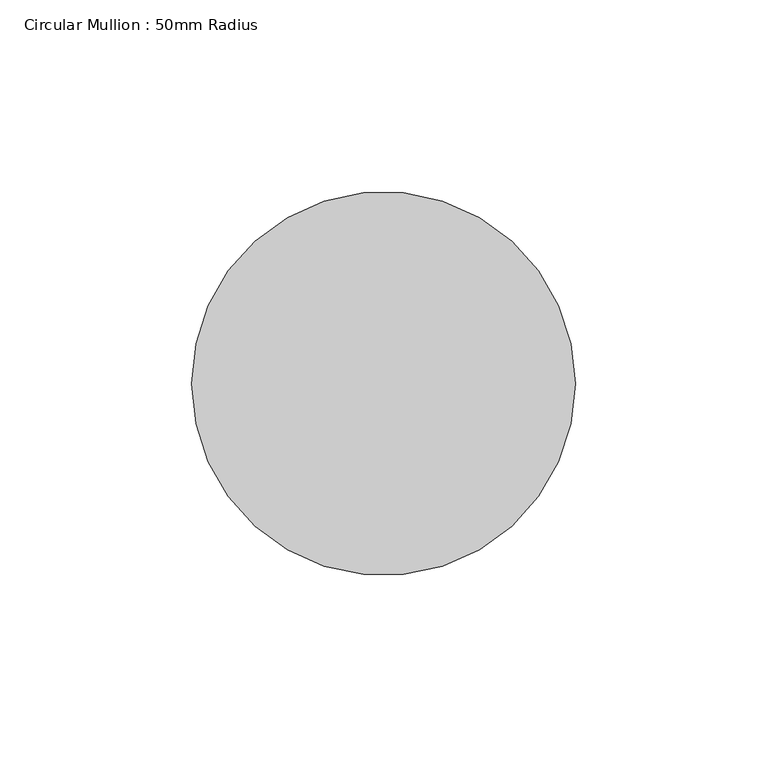
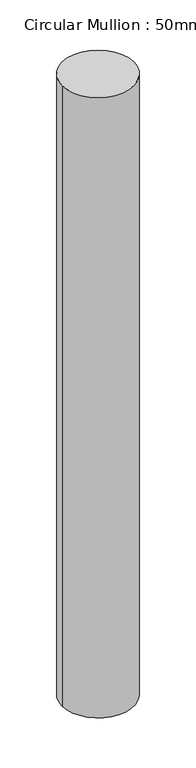
"""IFC4 building model written with IfcOpenShell, lengths in millimetres: member geometry, Circular Mullion : 50mm Radius."""

import ifcopenshell
import ifcopenshell.guid

model = None  # the IFC model being written
_history = None  # IfcOwnerHistory: only IFC2X3 demands one
_inside = {}  # id of a spatial element -> (the spatial element, [elements in it])
_under = {}  # id of a project, library or spatial element -> (it, [spatial elements below it])
_declared = {}  # id of a project -> (the project, [libraries it declares])
_typed = {}  # id of a type object -> (the type object, [elements of that type])
_made_of = {}  # id of a material, layer set ... -> (it, [elements and type objects made of it])


def new_model(schema):
    """Start an empty IFC model of exactly this schema.

    Asked for "IFC4X3", IfcOpenShell would pick the latest addendum, in which some entities
    have other attributes; the version numbers below select the first issue.
    IFC2X3 requires an IfcOwnerHistory on every rooted entity: one is made here for all.
    """
    global model, _history
    if schema == "IFC4X3":
        model = ifcopenshell.file(schema_version=(4, 3, 0, 0))
    else:
        model = ifcopenshell.file(schema=schema)
    _inside.clear()
    _under.clear()
    _declared.clear()
    _typed.clear()
    _made_of.clear()
    _history = None
    if model.schema == "IFC2X3":
        org = make("IfcOrganization", Name="unknown")
        user = make(
            "IfcPersonAndOrganization",
            ThePerson=make("IfcPerson", FamilyName="unknown"),
            TheOrganization=org,
        )
        app = make(
            "IfcApplication",
            ApplicationDeveloper=org,
            Version="unknown",
            ApplicationFullName="unknown",
            ApplicationIdentifier="unknown",
        )
        _history = make(
            "IfcOwnerHistory",
            OwningUser=user,
            OwningApplication=app,
            ChangeAction="ADDED",
            CreationDate=0,
        )
    return model


def make(cls, **values):
    """One entity of the class cls with the attributes given. An attribute that is None is left unset."""
    return model.create_entity(
        cls, **{name: value for name, value in values.items() if value is not None}
    )


def rooted(cls, **values):
    """An entity with a GlobalId (a new one), such as an element, a storey or a relation."""
    return make(cls, GlobalId=ifcopenshell.guid.new(), OwnerHistory=_history, **values)


def si_unit(unit_type, name, prefix=None):
    """IfcSIUnit, for example si_unit("LENGTHUNIT", "METRE", prefix="MILLI")."""
    return make("IfcSIUnit", UnitType=unit_type, Prefix=prefix, Name=name)


def assignment(units):
    """IfcUnitAssignment: the units of a project."""
    return None if units is None else make("IfcUnitAssignment", Units=units)


def point(xyz):
    """IfcCartesianPoint."""
    return None if xyz is None else make("IfcCartesianPoint", Coordinates=xyz)


def direction(xyz):
    """IfcDirection."""
    return None if xyz is None else make("IfcDirection", DirectionRatios=xyz)


def frame(location, z_axis=None, x_axis=None):
    """IfcAxis2Placement3D, a coordinate frame: its origin and axes. An axis left out is left unset."""
    return make(
        "IfcAxis2Placement3D",
        Location=point(location),
        Axis=direction(z_axis),
        RefDirection=direction(x_axis),
    )


def frame_2d(location, x_axis=None):
    """IfcAxis2Placement2D, a coordinate frame in the plane: its origin and x axis."""
    return make(
        "IfcAxis2Placement2D", Location=point(location), RefDirection=direction(x_axis)
    )


def origin():
    """The frame at (0, 0, 0) with its axes left unset."""
    return frame((0.0, 0.0, 0.0))


def origin_2d():
    """The frame at (0, 0) in the plane with its x axis left unset."""
    return frame_2d((0.0, 0.0))


def place(relative_to, where):
    """IfcLocalPlacement: puts the frame where relative to a parent placement (None: the world)."""
    return make(
        "IfcLocalPlacement", PlacementRelTo=relative_to, RelativePlacement=where
    )


def context(
    kind, dimensions, precision=None, world=None, true_north=None, identifier=None
):
    """IfcGeometricRepresentationContext, for example the 3D "Model" context."""
    return make(
        "IfcGeometricRepresentationContext",
        ContextIdentifier=identifier,
        ContextType=kind,
        CoordinateSpaceDimension=dimensions,
        Precision=precision,
        WorldCoordinateSystem=world,
        TrueNorth=true_north,
    )


def project(units=None, contexts=None):
    """IfcProject with its units and contexts."""
    return rooted(
        "IfcProject",
        Name="project",
        RepresentationContexts=contexts,
        UnitsInContext=assignment(units),
    )


def spatial(cls, under=None, at=None, **own):
    """A site, building, storey or space (cls), placed at a placement, below another one or the project."""
    s = rooted(cls, ObjectPlacement=at, **own)
    if under is not None:
        _under.setdefault(under.id(), (under, []))[1].append(s)
    return s


def circle_curve(where, radius):
    """IfcCircle in the frame where."""
    return make("IfcCircle", Position=where, Radius=radius)


def trimmed(basis, trim1, trim2, sense, master):
    """IfcTrimmedCurve: the piece of a basis curve between two trims."""
    return make(
        "IfcTrimmedCurve",
        BasisCurve=basis,
        Trim1=trim1,
        Trim2=trim2,
        SenseAgreement=sense,
        MasterRepresentation=master,
    )


def segment(curve, same_sense, transition):
    """IfcCompositeCurveSegment."""
    return make(
        "IfcCompositeCurveSegment",
        Transition=transition,
        SameSense=same_sense,
        ParentCurve=curve,
    )


def composite_curve(segments, self_intersect=None):
    """IfcCompositeCurve: segments joined end to end."""
    return make("IfcCompositeCurve", Segments=segments, SelfIntersect=self_intersect)


def outline(outer, holes=None, kind="AREA"):
    """IfcArbitraryClosedProfileDef: a profile drawn as a closed curve; with holes, ...WithVoids."""
    if holes is None:
        return make("IfcArbitraryClosedProfileDef", ProfileType=kind, OuterCurve=outer)
    return make(
        "IfcArbitraryProfileDefWithVoids",
        ProfileType=kind,
        OuterCurve=outer,
        InnerCurves=holes,
    )


def extrude(swept, where, along, depth):
    """IfcExtrudedAreaSolid: the profile swept, set in the frame where, extruded along a direction by depth."""
    return make(
        "IfcExtrudedAreaSolid",
        SweptArea=swept,
        Position=where,
        ExtrudedDirection=direction(along),
        Depth=depth,
    )


def shape(context_of_items, identifier, shape_type, items):
    """IfcShapeRepresentation: the items that make up one representation, for example the "Body"."""
    return make(
        "IfcShapeRepresentation",
        ContextOfItems=context_of_items,
        RepresentationIdentifier=identifier,
        RepresentationType=shape_type,
        Items=items,
    )


def source(mapping_origin, context_of_items, identifier, shape_type, items):
    """IfcRepresentationMap: a shape defined once, which mapped items show again and again."""
    return make(
        "IfcRepresentationMap",
        MappingOrigin=mapping_origin,
        MappedRepresentation=shape(context_of_items, identifier, shape_type, items),
    )


def transform(
    local_origin,
    x_axis=None,
    y_axis=None,
    z_axis=None,
    scale=None,
    scale2=None,
    scale3=None,
    uniform=True,
):
    """IfcCartesianTransformationOperator3D, or its non-uniform kind. x_axis, y_axis, z_axis: its Axis1, 2, 3."""
    if uniform:
        return make(
            "IfcCartesianTransformationOperator3D",
            Axis1=direction(x_axis),
            Axis2=direction(y_axis),
            LocalOrigin=point(local_origin),
            Scale=scale,
            Axis3=direction(z_axis),
        )
    return make(
        "IfcCartesianTransformationOperator3DnonUniform",
        Axis1=direction(x_axis),
        Axis2=direction(y_axis),
        LocalOrigin=point(local_origin),
        Scale=scale,
        Axis3=direction(z_axis),
        Scale2=scale2,
        Scale3=scale3,
    )


def mapped(mapping_source, mapping_target):
    """IfcMappedItem: shows the shape of a source again, moved by a transform."""
    return make(
        "IfcMappedItem", MappingSource=mapping_source, MappingTarget=mapping_target
    )


def made_of(thing, what):
    """Note that an element or type object is made of a material, layer set ...; save() writes the relation."""
    if what is not None:
        _made_of.setdefault(what.id(), (what, []))[1].append(thing)
    return thing


def element(
    cls,
    number,
    at=None,
    inside=None,
    cuts=None,
    type_object=None,
    material=None,
    context=None,
    identifier="Body",
    shape_type=None,
    held_by="IfcProductDefinitionShape",
    body=None,
    shapes=None,
    **own,
):
    """One element of the class cls, such as IfcWall. Its Tag is "e" and its number.

    at: its placement. inside: the storey or other place that contains it. cuts: it is an
    opening in that element (IfcRelVoidsElement). A single representation is given by context,
    identifier, shape_type and body (its items); several are given by shapes. held_by: the class
    of the entity that holds the representations. save() writes the other relations.
    """
    e = rooted(cls, Tag="e%d" % number, ObjectPlacement=at, **own)
    if body is not None:
        shapes = [shape(context, identifier, shape_type, body)]
    if shapes is not None:
        e.Representation = make(held_by, Representations=shapes)
    if inside is not None:
        _inside.setdefault(inside.id(), (inside, []))[1].append(e)
    if cuts is not None:
        rooted(
            "IfcRelVoidsElement", RelatingBuildingElement=cuts, RelatedOpeningElement=e
        )
    if type_object is not None:
        _typed.setdefault(type_object.id(), (type_object, []))[1].append(e)
    return made_of(e, material)


def aggregate(whole, parts):
    """IfcRelAggregates: a whole, such as a stair, and the parts it consists of."""
    return rooted("IfcRelAggregates", RelatingObject=whole, RelatedObjects=parts)


def save(model, path):
    """Write the relations noted so far, then the file.

    IfcRelAggregates (storeys below a building ...), IfcRelContainedInSpatialStructure (elements
    in a storey), IfcRelDefinesByType, IfcRelAssociatesMaterial and IfcRelDeclares: one each for
    every whole, place, type object, material and project.
    """
    for whole, parts in _under.values():
        aggregate(whole, parts)
    for where, things in _inside.values():
        rooted(
            "IfcRelContainedInSpatialStructure",
            RelatedElements=things,
            RelatingStructure=where,
        )
    for kind, things in _typed.values():
        rooted("IfcRelDefinesByType", RelatedObjects=things, RelatingType=kind)
    for what, things in _made_of.values():
        rooted("IfcRelAssociatesMaterial", RelatedObjects=things, RelatingMaterial=what)
    for by, libraries in _declared.values():
        rooted("IfcRelDeclares", RelatingContext=by, RelatedDefinitions=libraries)
    model.write(path)


def circular_mullion_50mm_radius_9a7117b8(model_context):
    return source(origin(), model_context, "Body", "SweptSolid", [
        extrude(outline(composite_curve([segment(trimmed(circle_curve(origin_2d(), 50.0), [point((50.0, 0.0))], [point((-50.0, 0.0))], False, "CARTESIAN"), True, "CONTINUOUS"), segment(trimmed(circle_curve(origin_2d(), 50.0), [point((-50.0, 0.0))], [point((50.0, 0.0))], False, "CARTESIAN"), True, "CONTINUOUS")], self_intersect=False)), frame((0.0, 0.0, -914.6323245), z_axis=(0.0, 0.0, 1.0), x_axis=(1.0, 0.0, 0.0)), (0.0, 0.0, 1.0), 914.6323245),
    ])


if __name__ == "__main__":
    model = new_model("IFC4")
    model_context = context("Model", 3, world=origin())
    ifc_project = project(units=[si_unit("LENGTHUNIT", "METRE", prefix="MILLI")], contexts=[model_context])
    site = spatial("IfcSite", under=ifc_project)
    building = spatial("IfcBuilding", under=site)
    placement = place(None, origin())
    circular_mullion_50mm_radius_shape = circular_mullion_50mm_radius_9a7117b8(model_context)
    element("IfcMember", 1, ObjectType="Circular Mullion : 50mm Radius", at=placement, inside=building, context=model_context, shape_type="MappedRepresentation", body=[
        mapped(circular_mullion_50mm_radius_shape, transform((0.0, 0.0, 0.0), x_axis=(1.0, 0.0, 0.0), y_axis=(0.0, 1.0, 0.0), z_axis=(0.0, 0.0, 1.0))),
    ])
    save(model, "model.ifc")

# Revit data of these elements
# Type "Circular Mullion : 50mm Radius"
#   built-in parameter 1007350 = 0.164042 (stored number, unit not read)
# Element 1 (IfcMember, "Circular Mullion : 50mm Radius")
#   Materials on its faces: "Aluminium"
# Materials
#   "Aluminium": class "Metal", colour RGB 247 247 247, transparency 0, Description = "Aluminium 6061", Cost = 0
